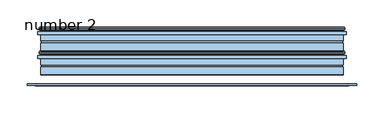
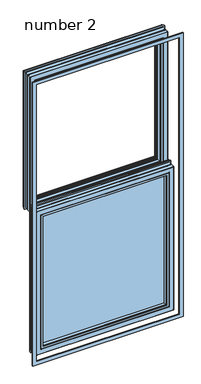
# IFC4 building model written with IfcOpenShell, lengths in millimetres: window geometry, Window-Exterior-Sierra-Double_Hung-Operating_Unit-18inch_48inch-Width-(Hi-Divide) : number 2.
# Revit data of these elements (continued)
# Type "Window-Exterior-Sierra-Double_Hung-Operating_Unit-18inch_48inch-Width-(Hi-Divide) : number 2" (continued)
#   Frame Height = 4' - 0"
#   First Simulite Width = 0' - 6.54167"
#   Default Sill Height = 3' - 0"
#   Actual Width = 2' - 0"
#   Actual Height = 4' - 0"
#   Actual Half Width = 1' - 0"
#   Actual Glass Width = 1' - 7 5/8"
#   Actual Glass Height = 1' - 8 1/2"
#   Wood Frame = yes
#   Total Number of Lites Per Panel = 4
#   Simulite Hi Divide Option = yes
#   Number of Vertical Simulites Greater than One = 2
#   Number of Hi Divide Verticals = 2
#   Clad Frame = no
#   Actual Vertical Simulites ( Hi Divide ) = 2
#   Vertical Simulite Type = element 491478
#   Interior Simulite = Wood - Sierra Pacific - Pine
#   Interior Panel Material = Wood - Sierra Pacific - Pine
#   Horizontal Simulite Type = element 491483
#   Glass = Glass - Sierra Doors - Clear
#   Frame = douglas fir
#   Exterior Simulite = Paint - Sierra Pacific - White 001
#   Exterior Panel Material = Paint - Sierra Pacific - White 001
#   Exterior Clad Material = Paint - Sierra Pacific - White 001
#   Wall Closure = (empty or 0)
# Element 1 (IfcWindow, "Window-Exterior-Sierra-Double_Hung-Operating_Unit-18inch_48inch-Width-(Hi-Divide) : number 2")
#   Materials on its faces: "Wood - Sierra Pacific - Pine", "Paint - Sierra Pacific - White 001", "douglas fir", "Glass - Sierra Doors - Clear"
# Materials
#   "Wood - Sierra Pacific - Pine": class "Miscellaneous", colour RGB 136 105 68, transparency 0
#   "Glass - Sierra Doors - Clear": class "Glass", colour RGB 0 0 255, transparency 0.75
#   "douglas fir": class "Generic", colour RGB 120 120 120, transparency 0, Cost = 0
#   "Paint - Sierra Pacific - White 001": class "Miscellaneous", colour RGB 111 112 111, transparency 0
